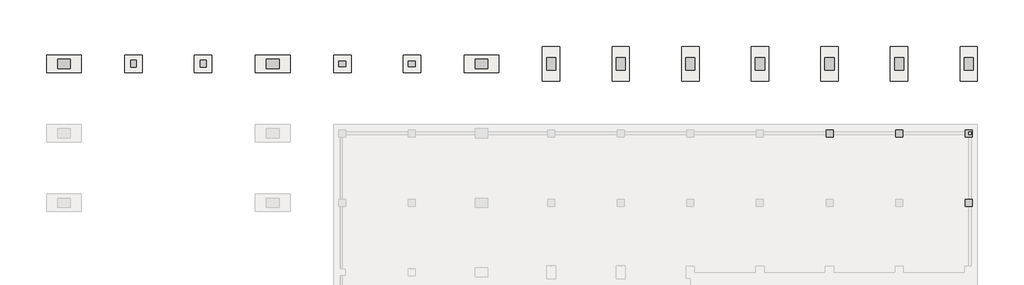
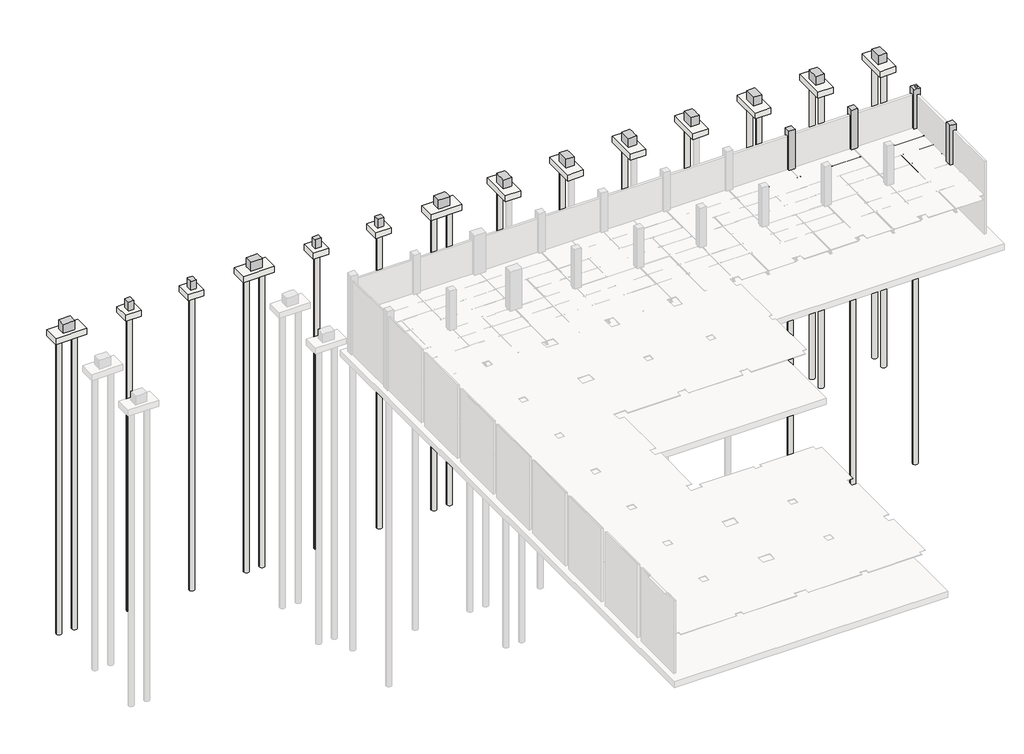
# Not in any storey, part 16 of 16: 37 slabs, 18 columns, 8 beams.
# Revit data of these elements (continued)
# Elements 41, 42, 43, 44, 45, 46, 47, 48, 49, 50, 51, 52, 53, 54, 55, 56, 57, 58, 59, 60 (IfcSlab, "PILE : H_SF_AR_S19_PHC Pile_Pre-boring_D500_L30")
#   Structural Material = Concrete, Precast
#   Phase Created = New Construction
#   Materials on its faces: "Concrete, Precast"
# Elements 61, 62, 63 (IfcSlab, "PILE : H_SF_AR_S19_PHC Pile_Pre-boring_D500_L30")
#   Structural Material = none
#   Phase Created = New Construction
# Materials
#   "Steel, 45-345": class "Metal", colour RGB 189 187 185, transparency 0, Description = "Steel 345 MPa", Cost = 0
#   "00_Concrete_Reinf. Conc.": class "Concrete", colour RGB 176 176 176, transparency 0, Description = "Reinf. Conc.", Cost = 0, Image = Concrete.Cast-In-Place.Flat.Polished.Grey.jpg
#   "Concrete, Precast": class "Concrete", colour RGB 115 116 108, transparency 0, Description = "Precast concrete", Cost = 0
